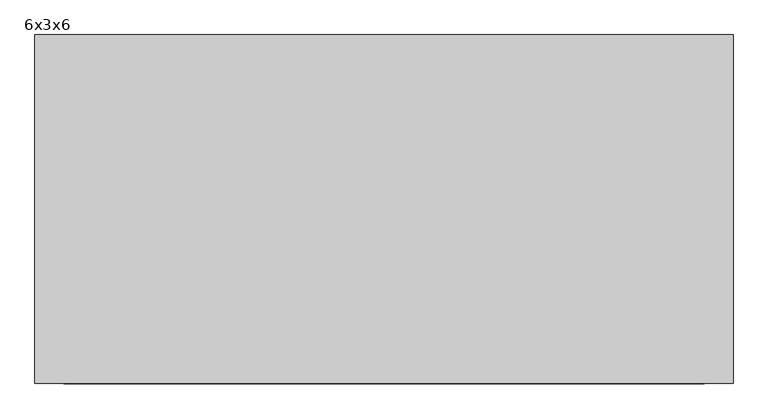
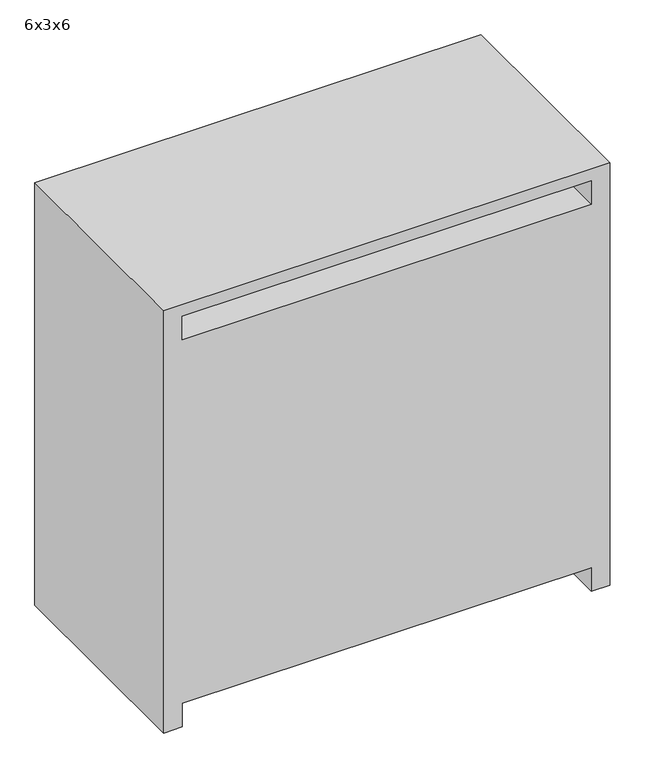
"""IFC4 building model written with IfcOpenShell, lengths in millimetres: proxy geometry, Transformer-Dry-Type-Siemens : 6x3x6."""

import ifcopenshell
import ifcopenshell.guid

model = None  # the IFC model being written
_history = None  # IfcOwnerHistory: only IFC2X3 demands one
_inside = {}  # id of a spatial element -> (the spatial element, [elements in it])
_under = {}  # id of a project, library or spatial element -> (it, [spatial elements below it])
_declared = {}  # id of a project -> (the project, [libraries it declares])
_typed = {}  # id of a type object -> (the type object, [elements of that type])
_made_of = {}  # id of a material, layer set ... -> (it, [elements and type objects made of it])


def new_model(schema):
    """Start an empty IFC model of exactly this schema.

    Asked for "IFC4X3", IfcOpenShell would pick the latest addendum, in which some entities
    have other attributes; the version numbers below select the first issue.
    IFC2X3 requires an IfcOwnerHistory on every rooted entity: one is made here for all.
    """
    global model, _history
    if schema == "IFC4X3":
        model = ifcopenshell.file(schema_version=(4, 3, 0, 0))
    else:
        model = ifcopenshell.file(schema=schema)
    _inside.clear()
    _under.clear()
    _declared.clear()
    _typed.clear()
    _made_of.clear()
    _history = None
    if model.schema == "IFC2X3":
        org = make("IfcOrganization", Name="unknown")
        user = make(
            "IfcPersonAndOrganization",
            ThePerson=make("IfcPerson", FamilyName="unknown"),
            TheOrganization=org,
        )
        app = make(
            "IfcApplication",
            ApplicationDeveloper=org,
            Version="unknown",
            ApplicationFullName="unknown",
            ApplicationIdentifier="unknown",
        )
        _history = make(
            "IfcOwnerHistory",
            OwningUser=user,
            OwningApplication=app,
            ChangeAction="ADDED",
            CreationDate=0,
        )
    return model


def make(cls, **values):
    """One entity of the class cls with the attributes given. An attribute that is None is left unset."""
    return model.create_entity(
        cls, **{name: value for name, value in values.items() if value is not None}
    )


def rooted(cls, **values):
    """An entity with a GlobalId (a new one), such as an element, a storey or a relation."""
    return make(cls, GlobalId=ifcopenshell.guid.new(), OwnerHistory=_history, **values)


def si_unit(unit_type, name, prefix=None):
    """IfcSIUnit, for example si_unit("LENGTHUNIT", "METRE", prefix="MILLI")."""
    return make("IfcSIUnit", UnitType=unit_type, Prefix=prefix, Name=name)


def assignment(units):
    """IfcUnitAssignment: the units of a project."""
    return None if units is None else make("IfcUnitAssignment", Units=units)


def point(xyz):
    """IfcCartesianPoint."""
    return None if xyz is None else make("IfcCartesianPoint", Coordinates=xyz)


def direction(xyz):
    """IfcDirection."""
    return None if xyz is None else make("IfcDirection", DirectionRatios=xyz)


def frame(location, z_axis=None, x_axis=None):
    """IfcAxis2Placement3D, a coordinate frame: its origin and axes. An axis left out is left unset."""
    return make(
        "IfcAxis2Placement3D",
        Location=point(location),
        Axis=direction(z_axis),
        RefDirection=direction(x_axis),
    )


def origin():
    """The frame at (0, 0, 0) with its axes left unset."""
    return frame((0.0, 0.0, 0.0))


def place(relative_to, where):
    """IfcLocalPlacement: puts the frame where relative to a parent placement (None: the world)."""
    return make(
        "IfcLocalPlacement", PlacementRelTo=relative_to, RelativePlacement=where
    )


def context(
    kind, dimensions, precision=None, world=None, true_north=None, identifier=None
):
    """IfcGeometricRepresentationContext, for example the 3D "Model" context."""
    return make(
        "IfcGeometricRepresentationContext",
        ContextIdentifier=identifier,
        ContextType=kind,
        CoordinateSpaceDimension=dimensions,
        Precision=precision,
        WorldCoordinateSystem=world,
        TrueNorth=true_north,
    )


def project(units=None, contexts=None):
    """IfcProject with its units and contexts."""
    return rooted(
        "IfcProject",
        Name="project",
        RepresentationContexts=contexts,
        UnitsInContext=assignment(units),
    )


def spatial(cls, under=None, at=None, **own):
    """A site, building, storey or space (cls), placed at a placement, below another one or the project."""
    s = rooted(cls, ObjectPlacement=at, **own)
    if under is not None:
        _under.setdefault(under.id(), (under, []))[1].append(s)
    return s


def polyline(points):
    """IfcPolyline through the points."""
    return make("IfcPolyline", Points=[point(p) for p in points])


def outline(outer, holes=None, kind="AREA"):
    """IfcArbitraryClosedProfileDef: a profile drawn as a closed curve; with holes, ...WithVoids."""
    if holes is None:
        return make("IfcArbitraryClosedProfileDef", ProfileType=kind, OuterCurve=outer)
    return make(
        "IfcArbitraryProfileDefWithVoids",
        ProfileType=kind,
        OuterCurve=outer,
        InnerCurves=holes,
    )


def extrude(swept, where, along, depth):
    """IfcExtrudedAreaSolid: the profile swept, set in the frame where, extruded along a direction by depth."""
    return make(
        "IfcExtrudedAreaSolid",
        SweptArea=swept,
        Position=where,
        ExtrudedDirection=direction(along),
        Depth=depth,
    )


def shape(context_of_items, identifier, shape_type, items):
    """IfcShapeRepresentation: the items that make up one representation, for example the "Body"."""
    return make(
        "IfcShapeRepresentation",
        ContextOfItems=context_of_items,
        RepresentationIdentifier=identifier,
        RepresentationType=shape_type,
        Items=items,
    )


def source(mapping_origin, context_of_items, identifier, shape_type, items):
    """IfcRepresentationMap: a shape defined once, which mapped items show again and again."""
    return make(
        "IfcRepresentationMap",
        MappingOrigin=mapping_origin,
        MappedRepresentation=shape(context_of_items, identifier, shape_type, items),
    )


def transform(
    local_origin,
    x_axis=None,
    y_axis=None,
    z_axis=None,
    scale=None,
    scale2=None,
    scale3=None,
    uniform=True,
):
    """IfcCartesianTransformationOperator3D, or its non-uniform kind. x_axis, y_axis, z_axis: its Axis1, 2, 3."""
    if uniform:
        return make(
            "IfcCartesianTransformationOperator3D",
            Axis1=direction(x_axis),
            Axis2=direction(y_axis),
            LocalOrigin=point(local_origin),
            Scale=scale,
            Axis3=direction(z_axis),
        )
    return make(
        "IfcCartesianTransformationOperator3DnonUniform",
        Axis1=direction(x_axis),
        Axis2=direction(y_axis),
        LocalOrigin=point(local_origin),
        Scale=scale,
        Axis3=direction(z_axis),
        Scale2=scale2,
        Scale3=scale3,
    )


def mapped(mapping_source, mapping_target):
    """IfcMappedItem: shows the shape of a source again, moved by a transform."""
    return make(
        "IfcMappedItem", MappingSource=mapping_source, MappingTarget=mapping_target
    )


def made_of(thing, what):
    """Note that an element or type object is made of a material, layer set ...; save() writes the relation."""
    if what is not None:
        _made_of.setdefault(what.id(), (what, []))[1].append(thing)
    return thing


def element(
    cls,
    number,
    at=None,
    inside=None,
    cuts=None,
    type_object=None,
    material=None,
    context=None,
    identifier="Body",
    shape_type=None,
    held_by="IfcProductDefinitionShape",
    body=None,
    shapes=None,
    **own,
):
    """One element of the class cls, such as IfcWall. Its Tag is "e" and its number.

    at: its placement. inside: the storey or other place that contains it. cuts: it is an
    opening in that element (IfcRelVoidsElement). A single representation is given by context,
    identifier, shape_type and body (its items); several are given by shapes. held_by: the class
    of the entity that holds the representations. save() writes the other relations.
    """
    e = rooted(cls, Tag="e%d" % number, ObjectPlacement=at, **own)
    if body is not None:
        shapes = [shape(context, identifier, shape_type, body)]
    if shapes is not None:
        e.Representation = make(held_by, Representations=shapes)
    if inside is not None:
        _inside.setdefault(inside.id(), (inside, []))[1].append(e)
    if cuts is not None:
        rooted(
            "IfcRelVoidsElement", RelatingBuildingElement=cuts, RelatedOpeningElement=e
        )
    if type_object is not None:
        _typed.setdefault(type_object.id(), (type_object, []))[1].append(e)
    return made_of(e, material)


def aggregate(whole, parts):
    """IfcRelAggregates: a whole, such as a stair, and the parts it consists of."""
    return rooted("IfcRelAggregates", RelatingObject=whole, RelatedObjects=parts)


def save(model, path):
    """Write the relations noted so far, then the file.

    IfcRelAggregates (storeys below a building ...), IfcRelContainedInSpatialStructure (elements
    in a storey), IfcRelDefinesByType, IfcRelAssociatesMaterial and IfcRelDeclares: one each for
    every whole, place, type object, material and project.
    """
    for whole, parts in _under.values():
        aggregate(whole, parts)
    for where, things in _inside.values():
        rooted(
            "IfcRelContainedInSpatialStructure",
            RelatedElements=things,
            RelatingStructure=where,
        )
    for kind, things in _typed.values():
        rooted("IfcRelDefinesByType", RelatedObjects=things, RelatingType=kind)
    for what, things in _made_of.values():
        rooted("IfcRelAssociatesMaterial", RelatedObjects=things, RelatingMaterial=what)
    for by, libraries in _declared.values():
        rooted("IfcRelDeclares", RelatingContext=by, RelatedDefinitions=libraries)
    model.write(path)


def proxy_6x3x6_82179be8(model_context):
    return source(origin(), model_context, "Body", "SweptSolid", [
        extrude(outline(polyline([(1828.8, 914.4), (1828.8, -914.4), (0.0, -914.4), (0.0, -838.2), (101.6, -838.2), (101.6, 838.2), (0.0, 838.2), (0.0, 914.4), (1828.8, 914.4)]), holes=[polyline([(1778.0, 838.2), (1676.4, 838.2), (1676.4, -838.2), (1778.0, -838.2), (1778.0, 838.2)])]), frame((0.0, -457.2, 0.0), z_axis=(0.0, 1.0, 0.0), x_axis=(0.0, 0.0, 1.0)), (0.0, 0.0, 1.0), 914.4),
    ])


if __name__ == "__main__":
    model = new_model("IFC4")
    model_context = context("Model", 3, world=origin())
    ifc_project = project(units=[si_unit("LENGTHUNIT", "METRE", prefix="MILLI")], contexts=[model_context])
    site = spatial("IfcSite", under=ifc_project)
    building = spatial("IfcBuilding", under=site)
    placement = place(None, origin())
    proxy_6x3x6_shape = proxy_6x3x6_82179be8(model_context)
    element("IfcBuildingElementProxy", 1, Name="Transformer-Dry-Type-Siemens : 6x3x6", ObjectType="Transformer-Dry-Type-Siemens : 6x3x6", at=placement, inside=building, context=model_context, shape_type="MappedRepresentation", body=[
        mapped(proxy_6x3x6_shape, transform((0.0, 0.0, 0.0), x_axis=(1.0, 0.0, 0.0), y_axis=(0.0, 1.0, 0.0), z_axis=(0.0, 0.0, 1.0))),
    ])
    save(model, "model.ifc")

# Revit data of these elements
# Type "Transformer-Dry-Type-Siemens : 6x3x6"
#   Weight = "5500"
#   Wattage = "DO NOT USE"
#   Voltage = "DO NOT USE"
#   URL = "http://www.usa.siemens.com/ce"
#   Transformer Material = "Aluminum"
#   Product Page URL = "http://www.sea.siemens.com/us/Products/PowerDistribution/Product/Transformers/Pages/Transformers.aspx"
#   Product Documentation Link = "http://www.sea.siemens.com/us/internet-dms/Internet/ConsultingEngineersComm/General/Docs/drytrans.pdf"
#   Model = "3F3Y015K13TP1"
#   Manufacturer = "Siemens Industry"
#   KVA = "750"
#   K Factor = "13"
#   Description = "Transformer"
#   Deg Rise = "150"
#   Copyright © = "© Siemens Industry, Inc. 2011"
#   CTRL Connector Description = "Equipment Power"
#   BOM URL [instance default] = ""
#   Assembly Code = "D5090900"
#   clearance = 3' - 0"
#   Width = 6' - 0"
#   Primary Voltage = 480 V
#   Power Factor = 1
#   Height = 6' - 0"
#   Depth = 3' - 0"
#   Apparent Load [instance default] = 0 VA
#   Has Not Contacted Siemens For Configuration [instance default] = no
#   Contacted Siemens For Configuration [instance default] = yes
#   Text Material = Paint- Siemens - Dark
#   Frame Material = Metal - Siemens - Steel
# Element 1 (IfcBuildingElementProxy, "Transformer-Dry-Type-Siemens : 6x3x6")
#   Materials on its faces: "Metal - Siemens - Steel"
# Materials
#   "Paint- Siemens - Dark": class "Metal", colour RGB 175 38 68, transparency 0
#   "Metal - Siemens - Steel": class "Metal", colour RGB 63 114 97, transparency 0, Cost = 0
